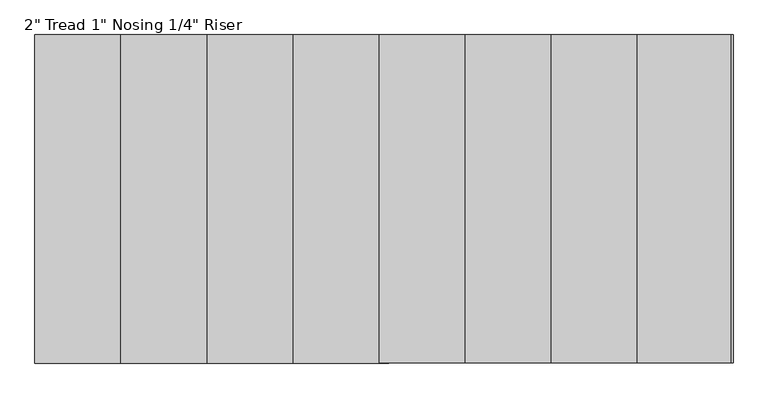
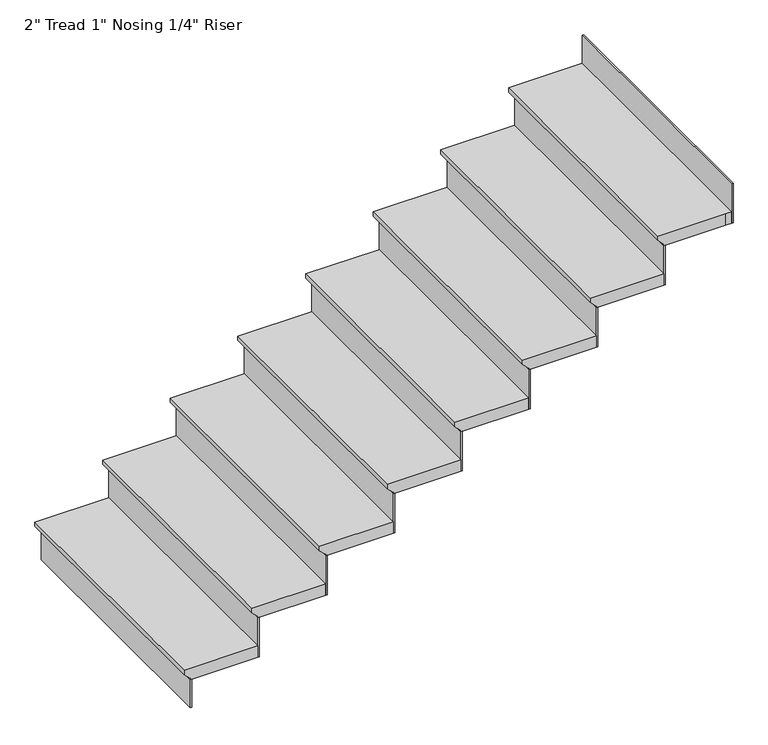
"""IFC4 building model written with IfcOpenShell, lengths in millimetres: stair flight geometry."""

from ifc_helpers import new_model, si_unit, origin, place, context, project, spatial, faceted_brep, source, transform, mapped, element, save


def stair_flight_0f12e121(model_context):
    return source(origin(), model_context, "Body", "Brep", [
        faceted_brep([(663721.188677, -551651.2413841, 153.9445946), (663721.188677, -551651.2413841, 172.9945946), (663721.188677, -550584.4413841, 172.9945946), (663721.188677, -550584.4413841, 153.9445946), (663746.588677, -551651.2413841, 128.5445946), (663746.588677, -550584.4413841, 128.5445946), (664025.988677, -551651.2413841, 172.9945946), (664025.988677, -550584.4413841, 172.9945946), (663746.588677, -550584.4413841, 122.1945946), (664025.988677, -550584.4413841, 122.1945946), (664025.988677, -551651.2413841, 122.1945946), (663746.588677, -551651.2413841, 122.1945946)], [[[0, 1, 2, 3]], [[4, 0, 3, 5]], [[2, 1, 6, 7]], [[8, 9, 10, 11]], [[2, 7, 9, 8, 5, 3]], [[8, 11, 4, 5]], [[6, 1, 0, 4, 11, 10]], [[7, 6, 10, 9]]]),
        faceted_brep([(663746.588677, -551651.2413841, 122.1945946), (663746.588677, -551651.2413841, 0.0), (663752.938677, -551651.2413841, 0.0), (663752.938677, -551651.2413841, 122.1945946), (663746.588677, -550584.4413841, 122.1945946), (663752.938677, -550584.4413841, 122.1945946), (663752.938677, -550584.4413841, 0.0), (663746.588677, -550584.4413841, 0.0)], [[[0, 1, 2, 3]], [[4, 5, 6, 7]], [[1, 0, 4, 7]], [[2, 1, 7, 6]], [[3, 2, 6, 5]], [[0, 3, 5, 4]]]),
        faceted_brep([(664025.988677, -551651.2413841, 295.1891892), (664025.988677, -551651.2413841, 122.1945946), (664032.338677, -551651.2413841, 122.1945946), (664032.338677, -551651.2413841, 295.1891892), (664025.988677, -550584.4413841, 295.1891892), (664032.338677, -550584.4413841, 295.1891892), (664032.338677, -550584.4413841, 122.1945946), (664025.988677, -550584.4413841, 122.1945946)], [[[0, 1, 2, 3]], [[4, 5, 6, 7]], [[1, 0, 4, 7]], [[2, 1, 7, 6]], [[3, 2, 6, 5]], [[0, 3, 5, 4]]]),
        faceted_brep([(664000.588677, -550584.4413841, 345.9891892), (664000.588677, -551651.2413841, 345.9891892), (664305.388677, -551651.2413841, 345.9891892), (664305.388677, -550584.4413841, 345.9891892), (664025.988677, -550584.4413841, 295.1891892), (664305.388677, -550584.4413841, 295.1891892), (664305.388677, -551651.2413841, 295.1891892), (664025.988677, -551651.2413841, 295.1891892), (664025.988677, -550584.4413841, 301.5391892), (664000.588677, -550584.4413841, 326.9391892), (664025.988677, -551651.2413841, 301.5391892), (664000.588677, -551651.2413841, 326.9391892)], [[[0, 1, 2, 3]], [[4, 5, 6, 7]], [[0, 3, 5, 4, 8, 9]], [[4, 7, 10, 8]], [[2, 1, 11, 10, 7, 6]], [[3, 2, 6, 5]], [[11, 1, 0, 9]], [[10, 11, 9, 8]]]),
        faceted_brep([(664305.388677, -551651.2413841, 468.1837838), (664305.388677, -551651.2413841, 295.1891892), (664311.738677, -551651.2413841, 295.1891892), (664311.738677, -551651.2413841, 468.1837838), (664305.388677, -550584.4413841, 468.1837838), (664311.738677, -550584.4413841, 468.1837838), (664311.738677, -550584.4413841, 295.1891892), (664305.388677, -550584.4413841, 295.1891892)], [[[0, 1, 2, 3]], [[4, 5, 6, 7]], [[1, 0, 4, 7]], [[2, 1, 7, 6]], [[3, 2, 6, 5]], [[0, 3, 5, 4]]]),
        faceted_brep([(664279.988677, -550584.4413841, 518.9837838), (664279.988677, -551651.2413841, 518.9837838), (664584.788677, -551651.2413841, 518.9837838), (664584.788677, -550584.4413841, 518.9837838), (664305.388677, -550584.4413841, 468.1837838), (664584.788677, -550584.4413841, 468.1837838), (664584.788677, -551651.2413841, 468.1837838), (664305.388677, -551651.2413841, 468.1837838), (664305.388677, -550584.4413841, 474.5337838), (664279.988677, -550584.4413841, 499.9337838), (664305.388677, -551651.2413841, 474.5337838), (664279.988677, -551651.2413841, 499.9337838)], [[[0, 1, 2, 3]], [[4, 5, 6, 7]], [[0, 3, 5, 4, 8, 9]], [[4, 7, 10, 8]], [[2, 1, 11, 10, 7, 6]], [[3, 2, 6, 5]], [[11, 1, 0, 9]], [[10, 11, 9, 8]]]),
        faceted_brep([(664584.788677, -551651.2413841, 641.1783784), (664584.788677, -551651.2413841, 468.1837838), (664591.138677, -551651.2413841, 468.1837838), (664591.138677, -551651.2413841, 641.1783784), (664584.788677, -550584.4413841, 641.1783784), (664591.138677, -550584.4413841, 641.1783784), (664591.138677, -550584.4413841, 468.1837838), (664584.788677, -550584.4413841, 468.1837838)], [[[0, 1, 2, 3]], [[4, 5, 6, 7]], [[1, 0, 4, 7]], [[2, 1, 7, 6]], [[3, 2, 6, 5]], [[0, 3, 5, 4]]]),
        faceted_brep([(664559.388677, -550584.4413841, 691.9783784), (664559.388677, -551651.2413841, 691.9783784), (664864.188677, -551651.2413841, 691.9783784), (664864.188677, -550584.4413841, 691.9783784), (664584.788677, -550584.4413841, 641.1783784), (664864.188677, -550584.4413841, 641.1783784), (664864.188677, -551651.2413841, 641.1783784), (664584.788677, -551651.2413841, 641.1783784), (664584.788677, -550584.4413841, 647.5283784), (664559.388677, -550584.4413841, 672.9283784), (664584.788677, -551651.2413841, 647.5283784), (664559.388677, -551651.2413841, 672.9283784)], [[[0, 1, 2, 3]], [[4, 5, 6, 7]], [[0, 3, 5, 4, 8, 9]], [[4, 7, 10, 8]], [[2, 1, 11, 10, 7, 6]], [[3, 2, 6, 5]], [[11, 1, 0, 9]], [[10, 11, 9, 8]]]),
        faceted_brep([(664864.188677, -551651.2413841, 814.172973), (664864.188677, -551651.2413841, 641.1783784), (664870.538677, -551651.2413841, 641.1783784), (664870.538677, -551651.2413841, 814.172973), (664864.188677, -550584.4413841, 814.172973), (664870.538677, -550584.4413841, 814.172973), (664870.538677, -550584.4413841, 641.1783784), (664864.188677, -550584.4413841, 641.1783784)], [[[0, 1, 2, 3]], [[4, 5, 6, 7]], [[1, 0, 4, 7]], [[2, 1, 7, 6]], [[3, 2, 6, 5]], [[0, 3, 5, 4]]]),
        faceted_brep([(664838.788677, -550584.4413841, 864.972973), (664838.788677, -551651.2413841, 864.972973), (665143.588677, -551651.2413841, 864.972973), (665143.588677, -550584.4413841, 864.972973), (664864.188677, -550584.4413841, 814.172973), (665143.588677, -550584.4413841, 814.172973), (665143.588677, -551651.2413841, 814.172973), (664864.188677, -551651.2413841, 814.172973), (664864.188677, -550584.4413841, 820.522973), (664838.788677, -550584.4413841, 845.922973), (664864.188677, -551651.2413841, 820.522973), (664838.788677, -551651.2413841, 845.922973)], [[[0, 1, 2, 3]], [[4, 5, 6, 7]], [[0, 3, 5, 4, 8, 9]], [[4, 7, 10, 8]], [[2, 1, 11, 10, 7, 6]], [[3, 2, 6, 5]], [[11, 1, 0, 9]], [[10, 11, 9, 8]]]),
        faceted_brep([(665143.588677, -551651.2413841, 987.1675676), (665143.588677, -551651.2413841, 814.172973), (665149.938677, -551651.2413841, 814.172973), (665149.938677, -551651.2413841, 987.1675676), (665143.588677, -550584.4413841, 987.1675676), (665149.938677, -550584.4413841, 987.1675676), (665149.938677, -550584.4413841, 814.172973), (665143.588677, -550584.4413841, 814.172973)], [[[0, 1, 2, 3]], [[4, 5, 6, 7]], [[1, 0, 4, 7]], [[2, 1, 7, 6]], [[3, 2, 6, 5]], [[0, 3, 5, 4]]]),
        faceted_brep([(665118.188677, -550584.4413841, 1037.9675676), (665118.188677, -551651.2413841, 1037.9675676), (665422.988677, -551651.2413841, 1037.9675676), (665422.988677, -550584.4413841, 1037.9675676), (665143.588677, -550584.4413841, 987.1675676), (665422.988677, -550584.4413841, 987.1675676), (665422.988677, -551651.2413841, 987.1675676), (665143.588677, -551651.2413841, 987.1675676), (665143.588677, -550584.4413841, 993.5175676), (665118.188677, -550584.4413841, 1018.9175676), (665143.588677, -551651.2413841, 993.5175676), (665118.188677, -551651.2413841, 1018.9175676)], [[[0, 1, 2, 3]], [[4, 5, 6, 7]], [[0, 3, 5, 4, 8, 9]], [[4, 7, 10, 8]], [[2, 1, 11, 10, 7, 6]], [[3, 2, 6, 5]], [[11, 1, 0, 9]], [[10, 11, 9, 8]]]),
        faceted_brep([(665422.988677, -551651.2413841, 1160.1621622), (665422.988677, -551651.2413841, 987.1675676), (665429.338677, -551651.2413841, 987.1675676), (665429.338677, -551651.2413841, 1160.1621622), (665422.988677, -550584.4413841, 1160.1621622), (665429.338677, -550584.4413841, 1160.1621622), (665429.338677, -550584.4413841, 987.1675676), (665422.988677, -550584.4413841, 987.1675676)], [[[0, 1, 2, 3]], [[4, 5, 6, 7]], [[1, 0, 4, 7]], [[2, 1, 7, 6]], [[3, 2, 6, 5]], [[0, 3, 5, 4]]]),
        faceted_brep([(665397.588677, -550584.4413841, 1210.9621622), (665397.588677, -551651.2413841, 1210.9621622), (665702.388677, -551651.2413841, 1210.9621622), (665702.388677, -550584.4413841, 1210.9621622), (665422.988677, -550584.4413841, 1160.1621622), (665702.388677, -550584.4413841, 1160.1621622), (665702.388677, -551651.2413841, 1160.1621622), (665422.988677, -551651.2413841, 1160.1621622), (665422.988677, -550584.4413841, 1166.5121622), (665397.588677, -550584.4413841, 1191.9121622), (665422.988677, -551651.2413841, 1166.5121622), (665397.588677, -551651.2413841, 1191.9121622)], [[[0, 1, 2, 3]], [[4, 5, 6, 7]], [[0, 3, 5, 4, 8, 9]], [[4, 7, 10, 8]], [[2, 1, 11, 10, 7, 6]], [[3, 2, 6, 5]], [[11, 1, 0, 9]], [[10, 11, 9, 8]]]),
        faceted_brep([(665981.788677, -551651.2413841, 1506.1513514), (665981.788677, -551651.2413841, 1333.1567568), (665988.138677, -551651.2413841, 1333.1567568), (665988.138677, -551651.2413841, 1506.1513514), (665981.788677, -550584.4413841, 1506.1513514), (665988.138677, -550584.4413841, 1506.1513514), (665988.138677, -550584.4413841, 1333.1567568), (665981.788677, -550584.4413841, 1333.1567568)], [[[0, 1, 2, 3]], [[4, 5, 6, 7]], [[1, 0, 4, 7]], [[2, 1, 7, 6]], [[3, 2, 6, 5]], [[0, 3, 5, 4]]]),
        faceted_brep([(665702.388677, -551651.2413841, 1333.1567568), (665702.388677, -551651.2413841, 1160.1621622), (665708.738677, -551651.2413841, 1160.1621622), (665708.738677, -551651.2413841, 1333.1567568), (665702.388677, -550584.4413841, 1333.1567568), (665708.738677, -550584.4413841, 1333.1567568), (665708.738677, -550584.4413841, 1160.1621622), (665702.388677, -550584.4413841, 1160.1621622)], [[[0, 1, 2, 3]], [[4, 5, 6, 7]], [[1, 0, 4, 7]], [[2, 1, 7, 6]], [[3, 2, 6, 5]], [[0, 3, 5, 4]]]),
        faceted_brep([(665676.988677, -550584.4413841, 1383.9567568), (665676.988677, -551651.2413841, 1383.9567568), (665956.388677, -551651.2413841, 1383.9567568), (665981.788677, -551651.2413841, 1383.9567568), (665981.788677, -550584.4413841, 1383.9567568), (665702.388677, -550584.4413841, 1333.1567568), (665981.788677, -550584.4413841, 1333.1567568), (665981.788677, -551651.2413841, 1333.1567568), (665956.388677, -551651.2413841, 1333.1567568), (665702.388677, -551651.2413841, 1333.1567568), (665702.388677, -550584.4413841, 1339.5067568), (665676.988677, -550584.4413841, 1364.9067568), (665702.388677, -551651.2413841, 1339.5067568), (665676.988677, -551651.2413841, 1364.9067568)], [[[0, 1, 2, 3, 4]], [[5, 6, 7, 8, 9]], [[0, 4, 6, 5, 10, 11]], [[5, 9, 12, 10]], [[2, 1, 13, 12, 9, 8]], [[3, 2, 8, 7]], [[4, 3, 7, 6]], [[13, 1, 0, 11]], [[12, 13, 11, 10]]]),
    ])


if __name__ == "__main__":
    model = new_model("IFC4")
    model_context = context("Model", 3, world=origin())
    ifc_project = project(units=[si_unit("LENGTHUNIT", "METRE", prefix="MILLI")], contexts=[model_context])
    site = spatial("IfcSite", under=ifc_project)
    building = spatial("IfcBuilding", under=site)
    placement = place(None, origin())
    stair_flight_shape = stair_flight_0f12e121(model_context)
    element("IfcStairFlight", 1, ObjectType="2\" Tread 1\" Nosing 1/4\" Riser", at=placement, inside=building, context=model_context, shape_type="MappedRepresentation", body=[
        mapped(stair_flight_shape, transform((0.0, 0.0, 0.0), x_axis=(1.0, 0.0, 0.0), y_axis=(0.0, 1.0, 0.0), z_axis=(0.0, 0.0, 1.0))),
    ])
    save(model, "model.ifc")
